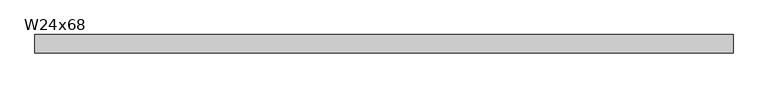
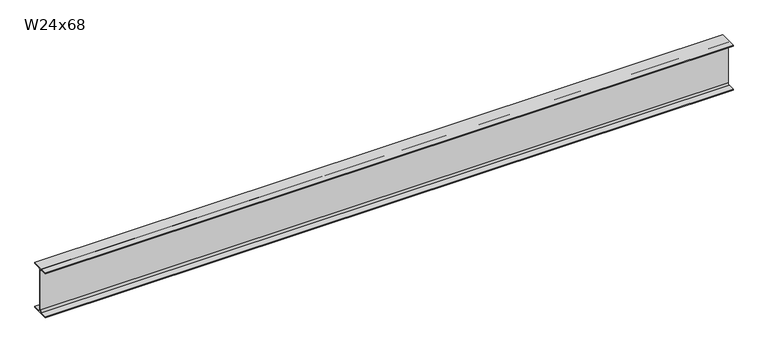
"""IFC4 building model written with IfcOpenShell, lengths in millimetres: beam geometry, RME W-Wide Flange : W24x68."""

from ifc_helpers import new_model, si_unit, point, frame, frame_2d, origin, place, context, project, spatial, polyline, circle_curve, trimmed, segment, composite_curve, outline, extrude, source, transform, mapped, element, save


def w24x68_3524241d(model_context):
    return source(origin(), model_context, "Body", "SweptSolid", [
        extrude(outline(composite_curve([segment(polyline([(113.919, -286.131), (113.919, -300.99), (-113.919, -300.99), (-113.919, -286.131), (-28.5115, -286.131)]), True, "CONTINUOUS"), segment(trimmed(circle_curve(frame_2d((-28.5115, -262.89)), 23.241), [point((-28.5115, -286.131))], [point((-5.2705, -262.89))], True, "CARTESIAN"), True, "CONTINUOUS"), segment(polyline([(-5.2705, -262.89), (-5.2705, 262.89)]), True, "CONTINUOUS"), segment(trimmed(circle_curve(frame_2d((-28.5115, 262.89)), 23.241), [point((-5.2705, 262.89))], [point((-28.5115, 286.131))], True, "CARTESIAN"), True, "CONTINUOUS"), segment(polyline([(-28.5115, 286.131), (-113.919, 286.131), (-113.919, 300.99), (113.919, 300.99), (113.919, 286.131), (28.5115, 286.131)]), True, "CONTINUOUS"), segment(trimmed(circle_curve(frame_2d((28.5115, 262.89)), 23.241), [point((28.5115, 286.131))], [point((5.2705, 262.89))], True, "CARTESIAN"), True, "CONTINUOUS"), segment(polyline([(5.2705, 262.89), (5.2705, -262.89)]), True, "CONTINUOUS"), segment(trimmed(circle_curve(frame_2d((28.5115, -262.89)), 23.241), [point((5.2705, -262.89))], [point((28.5115, -286.131))], True, "CARTESIAN"), True, "CONTINUOUS"), segment(polyline([(28.5115, -286.131), (113.919, -286.131)]), True, "CONTINUOUS")], self_intersect=False)), frame((-4339.0343748, 0.0, 0.0), z_axis=(1.0, 0.0, 0.0), x_axis=(0.0, 1.0, 0.0)), (0.0, 0.0, 1.0), 8678.9577497),
    ])


if __name__ == "__main__":
    model = new_model("IFC4")
    model_context = context("Model", 3, world=origin())
    ifc_project = project(units=[si_unit("LENGTHUNIT", "METRE", prefix="MILLI")], contexts=[model_context])
    site = spatial("IfcSite", under=ifc_project)
    building = spatial("IfcBuilding", under=site)
    placement = place(None, origin())
    w24x68_shape = w24x68_3524241d(model_context)
    element("IfcBeam", 1, ObjectType="RME W-Wide Flange : W24x68", at=placement, inside=building, context=model_context, shape_type="MappedRepresentation", body=[
        mapped(w24x68_shape, transform((0.0, 0.0, 0.0), x_axis=(1.0, 0.0, 0.0), y_axis=(0.0, 1.0, 0.0), z_axis=(0.0, 0.0, 1.0))),
    ])
    save(model, "model.ifc")

# Revit data of these elements
# Type "RME W-Wide Flange : W24x68"
#   WELD P [instance default] = ""
#   WELD LE [instance default] = ""
#   WELD D [instance default] = ""
#   TOP SECTION SIZE [instance default] = ""
#   TOP SECTION LENGTH [instance default] = ""
#   REMARKS [instance default] = ""
#   REINF TYPE [instance default] = ""
#   Nominal Size = "W24"
#   End Bearing Capacity [instance default] = ""
#   BOT SECTION SIZE [instance default] = ""
#   BOT SECTION LENGTH [instance default] = ""
#   Assembly Code = "B10"
#   W = 68
#   Start Extension Calculation [instance default] = 10' - 0"
#   Start Extension [instance default] = -0' - 0 1/2"
#   End Extension Calculation [instance default] = 10' - 0"
#   End Extension [instance default] = -0' - 0 1/2"
#   Length [instance default] = 5' - 0"
#   bf = 0' - 8.97"
#   d = 1' - 11.7"
#   k = 0' - 1 1/2"
#   k2 = 0' - 0.915"
#   tf = 0' - 0.585"
#   tw = 0' - 0.415"
#   A = 0.139583 SF
#   Structural Material [instance default] = Metal - Steel - ASTM A992
# Element 1 (IfcBeam, "RME W-Wide Flange : W24x68")
#   Length = 29' - 2 21/32"
#   Materials on its faces: "Metal - Steel - ASTM A992"
# Materials
#   "Metal - Steel - ASTM A992": class "Metal", colour RGB 255 128 0, transparency 0
